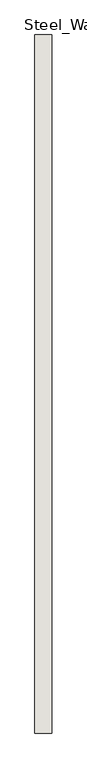
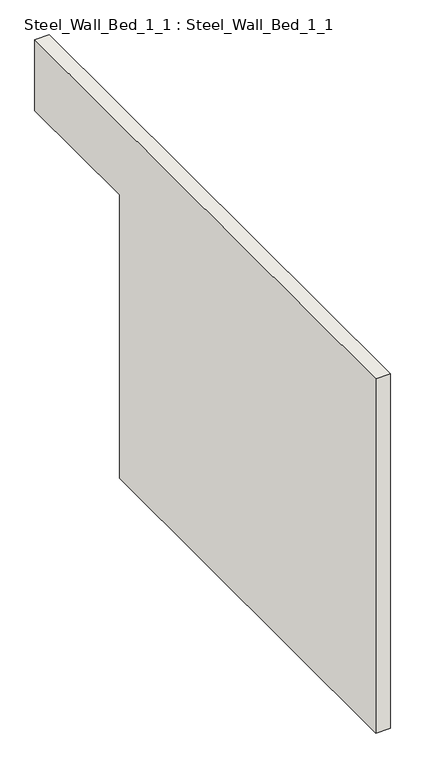
"""IFC4 building model written with IfcOpenShell, lengths in millimetres: wall geometry, Steel_Wall_Bed_1_1 : Steel_Wall_Bed_1_1."""

from ifc_helpers import new_model, si_unit, frame, origin, place, context, project, spatial, polyline, outline, extrude, source, transform, mapped, element, save


def steel_wall_bed_1_1_steel_wall_bed_1_1_07c56df4(model_context):
    return source(origin(), model_context, "Body", "SweptSolid", [
        extrude(outline(polyline([(495.0, 2850.0), (4595.0, 2850.0), (4595.0, 2330.0), (3575.0, 2330.0), (3575.0, 250.0), (495.0, 250.0), (495.0, 2850.0)])), frame((1950.0, 0.0, 0.0), z_axis=(1.0, 0.0, 0.0), x_axis=(0.0, 1.0, 0.0)), (0.0, 0.0, 1.0), 100.0),
    ])


if __name__ == "__main__":
    model = new_model("IFC4")
    model_context = context("Model", 3, world=origin())
    ifc_project = project(units=[si_unit("LENGTHUNIT", "METRE", prefix="MILLI")], contexts=[model_context])
    site = spatial("IfcSite", under=ifc_project)
    building = spatial("IfcBuilding", under=site)
    placement = place(None, origin())
    steel_wall_bed_1_1_steel_wall_bed_1_1_shape = steel_wall_bed_1_1_steel_wall_bed_1_1_07c56df4(model_context)
    element("IfcWall", 1, ObjectType="Steel_Wall_Bed_1_1 : Steel_Wall_Bed_1_1", at=placement, inside=building, context=model_context, shape_type="MappedRepresentation", body=[
        mapped(steel_wall_bed_1_1_steel_wall_bed_1_1_shape, transform((0.0, 0.0, 0.0), x_axis=(1.0, 0.0, 0.0), y_axis=(0.0, 1.0, 0.0), z_axis=(0.0, 0.0, 1.0))),
    ])
    save(model, "model.ifc")

# Revit data of these elements
# Type "Steel_Wall_Bed_1_1 : Steel_Wall_Bed_1_1"
#   NameOverride = "Steel_Wall_Bed_1_1"
# Element 1 (IfcWall, "Steel_Wall_Bed_1_1 : Steel_Wall_Bed_1_1")
#   Materials on its faces: "IfcSurfaceStyle #33"
# Materials
#   "IfcSurfaceStyle #33": class "Unassigned", colour RGB 214 214 214, transparency 0
